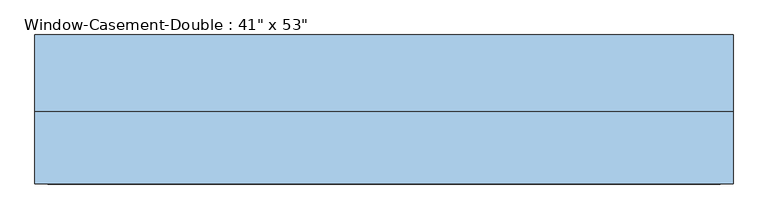
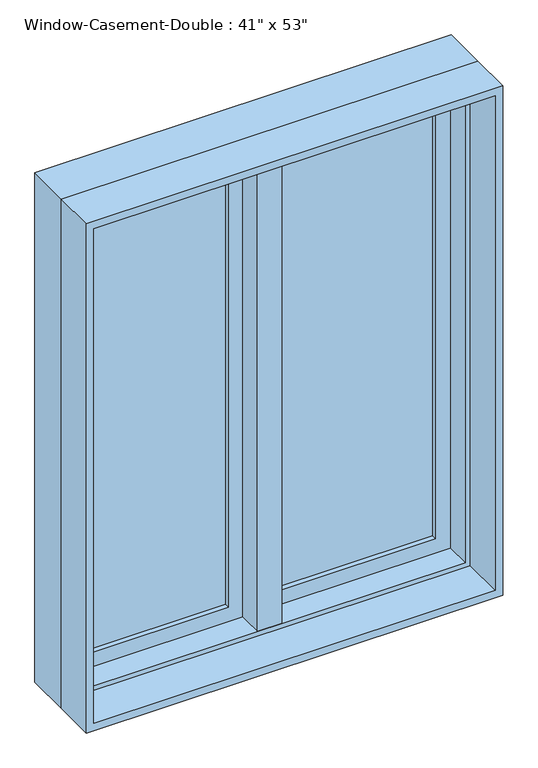
"""IFC4 building model written with IfcOpenShell, lengths in millimetres: window geometry."""

import ifcopenshell
import ifcopenshell.guid

model = None  # the IFC model being written
_history = None  # IfcOwnerHistory: only IFC2X3 demands one
_inside = {}  # id of a spatial element -> (the spatial element, [elements in it])
_under = {}  # id of a project, library or spatial element -> (it, [spatial elements below it])
_declared = {}  # id of a project -> (the project, [libraries it declares])
_typed = {}  # id of a type object -> (the type object, [elements of that type])
_made_of = {}  # id of a material, layer set ... -> (it, [elements and type objects made of it])


def new_model(schema):
    """Start an empty IFC model of exactly this schema.

    Asked for "IFC4X3", IfcOpenShell would pick the latest addendum, in which some entities
    have other attributes; the version numbers below select the first issue.
    IFC2X3 requires an IfcOwnerHistory on every rooted entity: one is made here for all.
    """
    global model, _history
    if schema == "IFC4X3":
        model = ifcopenshell.file(schema_version=(4, 3, 0, 0))
    else:
        model = ifcopenshell.file(schema=schema)
    _inside.clear()
    _under.clear()
    _declared.clear()
    _typed.clear()
    _made_of.clear()
    _history = None
    if model.schema == "IFC2X3":
        org = make("IfcOrganization", Name="unknown")
        user = make(
            "IfcPersonAndOrganization",
            ThePerson=make("IfcPerson", FamilyName="unknown"),
            TheOrganization=org,
        )
        app = make(
            "IfcApplication",
            ApplicationDeveloper=org,
            Version="unknown",
            ApplicationFullName="unknown",
            ApplicationIdentifier="unknown",
        )
        _history = make(
            "IfcOwnerHistory",
            OwningUser=user,
            OwningApplication=app,
            ChangeAction="ADDED",
            CreationDate=0,
        )
    return model


def make(cls, **values):
    """One entity of the class cls with the attributes given. An attribute that is None is left unset."""
    return model.create_entity(
        cls, **{name: value for name, value in values.items() if value is not None}
    )


def rooted(cls, **values):
    """An entity with a GlobalId (a new one), such as an element, a storey or a relation."""
    return make(cls, GlobalId=ifcopenshell.guid.new(), OwnerHistory=_history, **values)


def si_unit(unit_type, name, prefix=None):
    """IfcSIUnit, for example si_unit("LENGTHUNIT", "METRE", prefix="MILLI")."""
    return make("IfcSIUnit", UnitType=unit_type, Prefix=prefix, Name=name)


def assignment(units):
    """IfcUnitAssignment: the units of a project."""
    return None if units is None else make("IfcUnitAssignment", Units=units)


def point(xyz):
    """IfcCartesianPoint."""
    return None if xyz is None else make("IfcCartesianPoint", Coordinates=xyz)


def direction(xyz):
    """IfcDirection."""
    return None if xyz is None else make("IfcDirection", DirectionRatios=xyz)


def frame(location, z_axis=None, x_axis=None):
    """IfcAxis2Placement3D, a coordinate frame: its origin and axes. An axis left out is left unset."""
    return make(
        "IfcAxis2Placement3D",
        Location=point(location),
        Axis=direction(z_axis),
        RefDirection=direction(x_axis),
    )


def origin():
    """The frame at (0, 0, 0) with its axes left unset."""
    return frame((0.0, 0.0, 0.0))


def place(relative_to, where):
    """IfcLocalPlacement: puts the frame where relative to a parent placement (None: the world)."""
    return make(
        "IfcLocalPlacement", PlacementRelTo=relative_to, RelativePlacement=where
    )


def context(
    kind, dimensions, precision=None, world=None, true_north=None, identifier=None
):
    """IfcGeometricRepresentationContext, for example the 3D "Model" context."""
    return make(
        "IfcGeometricRepresentationContext",
        ContextIdentifier=identifier,
        ContextType=kind,
        CoordinateSpaceDimension=dimensions,
        Precision=precision,
        WorldCoordinateSystem=world,
        TrueNorth=true_north,
    )


def project(units=None, contexts=None):
    """IfcProject with its units and contexts."""
    return rooted(
        "IfcProject",
        Name="project",
        RepresentationContexts=contexts,
        UnitsInContext=assignment(units),
    )


def spatial(cls, under=None, at=None, **own):
    """A site, building, storey or space (cls), placed at a placement, below another one or the project."""
    s = rooted(cls, ObjectPlacement=at, **own)
    if under is not None:
        _under.setdefault(under.id(), (under, []))[1].append(s)
    return s


def polyline(points):
    """IfcPolyline through the points."""
    return make("IfcPolyline", Points=[point(p) for p in points])


def outline(outer, holes=None, kind="AREA"):
    """IfcArbitraryClosedProfileDef: a profile drawn as a closed curve; with holes, ...WithVoids."""
    if holes is None:
        return make("IfcArbitraryClosedProfileDef", ProfileType=kind, OuterCurve=outer)
    return make(
        "IfcArbitraryProfileDefWithVoids",
        ProfileType=kind,
        OuterCurve=outer,
        InnerCurves=holes,
    )


def extrude(swept, where, along, depth):
    """IfcExtrudedAreaSolid: the profile swept, set in the frame where, extruded along a direction by depth."""
    return make(
        "IfcExtrudedAreaSolid",
        SweptArea=swept,
        Position=where,
        ExtrudedDirection=direction(along),
        Depth=depth,
    )


def faces_of(points, faces, orient=None, outer=None):
    """IfcFace entities. A face is a list of loops; a loop is a list of indices into points, from 0.

    orient and outer hold one flag for each loop. By default every Orientation is true, the
    first loop of a face is its IfcFaceOuterBound and the others are IfcFaceBound.
    """
    made = []
    for i, loops in enumerate(faces):
        bounds = []
        for j, loop in enumerate(loops):
            is_outer = j == 0 if outer is None else outer[i][j]
            bounds.append(
                make(
                    "IfcFaceOuterBound" if is_outer else "IfcFaceBound",
                    Bound=make("IfcPolyLoop", Polygon=[points[k] for k in loop]),
                    Orientation=True if orient is None else orient[i][j],
                )
            )
        made.append(make("IfcFace", Bounds=bounds))
    return made


def faceted_brep(points, faces, orient=None, outer=None, voids=None):
    """IfcFacetedBrep: a solid bounded by flat faces; with voids (closed shells), ...WithVoids."""
    shared = [point(p) for p in points]
    hull = make("IfcClosedShell", CfsFaces=faces_of(shared, faces, orient, outer))
    if voids is None:
        return make("IfcFacetedBrep", Outer=hull)
    return make(
        "IfcFacetedBrepWithVoids",
        Outer=hull,
        Voids=[
            make(cls, CfsFaces=faces_of(shared, fs, o, b)) for cls, fs, o, b in voids
        ],
    )


def shape(context_of_items, identifier, shape_type, items):
    """IfcShapeRepresentation: the items that make up one representation, for example the "Body"."""
    return make(
        "IfcShapeRepresentation",
        ContextOfItems=context_of_items,
        RepresentationIdentifier=identifier,
        RepresentationType=shape_type,
        Items=items,
    )


def source(mapping_origin, context_of_items, identifier, shape_type, items):
    """IfcRepresentationMap: a shape defined once, which mapped items show again and again."""
    return make(
        "IfcRepresentationMap",
        MappingOrigin=mapping_origin,
        MappedRepresentation=shape(context_of_items, identifier, shape_type, items),
    )


def transform(
    local_origin,
    x_axis=None,
    y_axis=None,
    z_axis=None,
    scale=None,
    scale2=None,
    scale3=None,
    uniform=True,
):
    """IfcCartesianTransformationOperator3D, or its non-uniform kind. x_axis, y_axis, z_axis: its Axis1, 2, 3."""
    if uniform:
        return make(
            "IfcCartesianTransformationOperator3D",
            Axis1=direction(x_axis),
            Axis2=direction(y_axis),
            LocalOrigin=point(local_origin),
            Scale=scale,
            Axis3=direction(z_axis),
        )
    return make(
        "IfcCartesianTransformationOperator3DnonUniform",
        Axis1=direction(x_axis),
        Axis2=direction(y_axis),
        LocalOrigin=point(local_origin),
        Scale=scale,
        Axis3=direction(z_axis),
        Scale2=scale2,
        Scale3=scale3,
    )


def mapped(mapping_source, mapping_target):
    """IfcMappedItem: shows the shape of a source again, moved by a transform."""
    return make(
        "IfcMappedItem", MappingSource=mapping_source, MappingTarget=mapping_target
    )


def made_of(thing, what):
    """Note that an element or type object is made of a material, layer set ...; save() writes the relation."""
    if what is not None:
        _made_of.setdefault(what.id(), (what, []))[1].append(thing)
    return thing


def element(
    cls,
    number,
    at=None,
    inside=None,
    cuts=None,
    type_object=None,
    material=None,
    context=None,
    identifier="Body",
    shape_type=None,
    held_by="IfcProductDefinitionShape",
    body=None,
    shapes=None,
    **own,
):
    """One element of the class cls, such as IfcWall. Its Tag is "e" and its number.

    at: its placement. inside: the storey or other place that contains it. cuts: it is an
    opening in that element (IfcRelVoidsElement). A single representation is given by context,
    identifier, shape_type and body (its items); several are given by shapes. held_by: the class
    of the entity that holds the representations. save() writes the other relations.
    """
    e = rooted(cls, Tag="e%d" % number, ObjectPlacement=at, **own)
    if body is not None:
        shapes = [shape(context, identifier, shape_type, body)]
    if shapes is not None:
        e.Representation = make(held_by, Representations=shapes)
    if inside is not None:
        _inside.setdefault(inside.id(), (inside, []))[1].append(e)
    if cuts is not None:
        rooted(
            "IfcRelVoidsElement", RelatingBuildingElement=cuts, RelatedOpeningElement=e
        )
    if type_object is not None:
        _typed.setdefault(type_object.id(), (type_object, []))[1].append(e)
    return made_of(e, material)


def aggregate(whole, parts):
    """IfcRelAggregates: a whole, such as a stair, and the parts it consists of."""
    return rooted("IfcRelAggregates", RelatingObject=whole, RelatedObjects=parts)


def save(model, path):
    """Write the relations noted so far, then the file.

    IfcRelAggregates (storeys below a building ...), IfcRelContainedInSpatialStructure (elements
    in a storey), IfcRelDefinesByType, IfcRelAssociatesMaterial and IfcRelDeclares: one each for
    every whole, place, type object, material and project.
    """
    for whole, parts in _under.values():
        aggregate(whole, parts)
    for where, things in _inside.values():
        rooted(
            "IfcRelContainedInSpatialStructure",
            RelatedElements=things,
            RelatingStructure=where,
        )
    for kind, things in _typed.values():
        rooted("IfcRelDefinesByType", RelatedObjects=things, RelatingType=kind)
    for what, things in _made_of.values():
        rooted("IfcRelAssociatesMaterial", RelatedObjects=things, RelatingMaterial=what)
    for by, libraries in _declared.values():
        rooted("IfcRelDeclares", RelatingContext=by, RelatedDefinitions=libraries)
    model.write(path)


def window_0de3df1e(model_context):
    return source(origin(), model_context, "Body", "SolidModel", [
        faceted_brep([(9.525, 120.65, 2247.9), (-9.525, 120.65, 2247.9), (-9.525, 69.85, 2247.9), (9.525, 69.85, 2247.9), (9.525, 120.65, 927.1), (9.525, 69.85, 927.1), (-9.525, 69.85, 927.1), (-9.525, 120.65, 927.1), (-9.525, 69.85, 946.15), (-9.525, 69.85, 2228.85), (-30.1625, 69.85, 946.15), (-30.1625, 69.85, 2228.85), (-30.1625, 6.35, 946.15), (-30.1625, 6.35, 2228.85), (30.1625, 6.35, 946.15), (30.1625, 6.35, 2228.85), (30.1625, 69.85, 946.15), (30.1625, 69.85, 2228.85), (9.525, 69.85, 946.15), (9.525, 69.85, 2228.85)], [[[0, 1, 2, 3]], [[4, 5, 6, 7]], [[1, 0, 4, 7]], [[2, 1, 7, 6, 8, 9]], [[9, 8, 10, 11]], [[11, 10, 12, 13]], [[13, 12, 14, 15]], [[15, 14, 16, 17]], [[17, 16, 18, 19]], [[0, 3, 19, 18, 5, 4]], [[18, 8, 6, 5]], [[9, 19, 3, 2]], [[8, 18, 16, 14, 12, 10]], [[19, 9, 11, 13, 15, 17]]]),
        extrude(outline(polyline([(-66.675, 101.6), (-66.675, 95.25), (-450.85, 95.25), (-450.85, 101.6), (-66.675, 101.6)])), frame((0.0, 0.0, 984.25), z_axis=(0.0, 0.0, 1.0), x_axis=(1.0, 0.0, 0.0)), (0.0, 0.0, 1.0), 1206.5),
        extrude(outline(polyline([(-450.85, 82.55), (-450.85, 88.9), (-66.675, 88.9), (-66.675, 82.55), (-450.85, 82.55)])), frame((0.0, 0.0, 984.25), z_axis=(0.0, 0.0, 1.0), x_axis=(1.0, 0.0, 0.0)), (0.0, 0.0, 1.0), 1206.5),
        extrude(outline(polyline([(450.85, 101.6), (450.85, 95.25), (66.675, 95.25), (66.675, 101.6), (450.85, 101.6)])), frame((0.0, 0.0, 984.25), z_axis=(0.0, 0.0, 1.0), x_axis=(1.0, 0.0, 0.0)), (0.0, 0.0, 1.0), 1206.5),
        extrude(outline(polyline([(66.675, 82.55), (66.675, 88.9), (450.85, 88.9), (450.85, 82.55), (66.675, 82.55)])), frame((0.0, 0.0, 984.25), z_axis=(0.0, 0.0, 1.0), x_axis=(1.0, 0.0, 0.0)), (0.0, 0.0, 1.0), 1206.5),
        extrude(outline(polyline([(2247.9, -508.0), (927.1, -508.0), (927.1, -9.525), (2247.9, -9.525), (2247.9, -508.0)]), holes=[polyline([(2190.75, -66.675), (984.25, -66.675), (984.25, -450.85), (2190.75, -450.85), (2190.75, -66.675)])]), frame((0.0, 69.85, 0.0), z_axis=(0.0, 1.0, 0.0), x_axis=(0.0, 0.0, 1.0)), (0.0, 0.0, 1.0), 44.45),
        extrude(outline(polyline([(927.1, 508.0), (2247.9, 508.0), (2247.9, 9.525), (927.1, 9.525), (927.1, 508.0)]), holes=[polyline([(984.25, 66.675), (2190.75, 66.675), (2190.75, 450.85), (984.25, 450.85), (984.25, 66.675)])]), frame((0.0, 69.85, 0.0), z_axis=(0.0, 1.0, 0.0), x_axis=(0.0, 0.0, 1.0)), (0.0, 0.0, 1.0), 44.45),
        extrude(outline(polyline([(2260.6, -520.7), (914.4, -520.7), (914.4, 520.7), (2260.6, 520.7), (2260.6, -520.7)]), holes=[polyline([(2241.55, 501.65), (933.45, 501.65), (933.45, -501.65), (2241.55, -501.65), (2241.55, 501.65)])]), frame((0.0, -101.6, 0.0), z_axis=(0.0, 1.0, 0.0), x_axis=(0.0, 0.0, 1.0)), (0.0, 0.0, 1.0), 107.95),
        faceted_brep([(488.95, 69.85, 2228.85), (488.95, 6.35, 2228.85), (-488.95, 6.35, 2228.85), (-488.95, 69.85, 2228.85), (508.0, 120.65, 2247.9), (508.0, 69.85, 2247.9), (-508.0, 69.85, 2247.9), (-508.0, 120.65, 2247.9), (520.7, 6.35, 2260.6), (520.7, 120.65, 2260.6), (-520.7, 120.65, 2260.6), (-520.7, 6.35, 2260.6), (-488.95, 6.35, 946.15), (-488.95, 69.85, 946.15), (-508.0, 69.85, 927.1), (-508.0, 120.65, 927.1), (-520.7, 120.65, 914.4), (-520.7, 6.35, 914.4), (488.95, 6.35, 946.15), (488.95, 69.85, 946.15), (508.0, 69.85, 927.1), (508.0, 120.65, 927.1), (520.7, 120.65, 914.4), (520.7, 6.35, 914.4)], [[[0, 1, 2, 3]], [[4, 5, 6, 7]], [[8, 9, 10, 11]], [[3, 2, 12, 13]], [[7, 6, 14, 15]], [[11, 10, 16, 17]], [[13, 12, 18, 19]], [[15, 14, 20, 21]], [[17, 16, 22, 23]], [[11, 17, 23, 8], [1, 18, 12, 2]], [[19, 18, 1, 0]], [[5, 20, 14, 6], [3, 13, 19, 0]], [[21, 20, 5, 4]], [[23, 22, 9, 8]], [[9, 22, 16, 10], [7, 15, 21, 4]]]),
    ])


if __name__ == "__main__":
    model = new_model("IFC4")
    model_context = context("Model", 3, world=origin())
    ifc_project = project(units=[si_unit("LENGTHUNIT", "METRE", prefix="MILLI")], contexts=[model_context])
    site = spatial("IfcSite", under=ifc_project)
    building = spatial("IfcBuilding", under=site)
    placement = place(None, origin())
    window_shape = window_0de3df1e(model_context)
    element("IfcWindow", 1, ObjectType="Window-Casement-Double : 41\" x 53\"", at=placement, inside=building, context=model_context, shape_type="MappedRepresentation", body=[
        mapped(window_shape, transform((0.0, 0.0, 0.0), x_axis=(1.0, 0.0, 0.0), y_axis=(0.0, 1.0, 0.0), z_axis=(0.0, 0.0, 1.0))),
    ])
    save(model, "model.ifc")

# Revit data of these elements
# Type "Window-Casement-Double : 41\" x 53\""
#   Type Mark = "60"
#   Fire Rating = "0.5h"
#   Assembly Code = "B2020100"
#   Analytic Construction = "Double glazing - domestic"
#   Frame Extension [instance default] = 0' - 0 1/4"
#   Window Inset [instance default] = 0' - 0"
#   Wall Thickness [instance default] = 0' - 6"
#   Interior Wall Closure [instance default] = 0' - 2 1/4"
#   Half Width = 1' - 8 1/2"
#   Visual Light Transmittance = 0.81
#   Thermal Resistance (R) = 1.8146 (h·ft²·°F)/BTU
#   Solar Heat Gain Coefficient = 0.76
#   Rough Width = 3' - 5 1/2"
#   Rough Height = 4' - 5 1/2"
#   Height = 4' - 5"
#   Heat Transfer Coefficient (U) = 0.5511 BTU/(h·ft²·°F)
#   Exterior Wall Closure [instance default] = 0' - 1 1/4"
#   Extension Jamb [instance default] = 0' - 2 1/4"
#   Default Sill Height = 3' - 0"
#   Width = 3' - 5"
#   Define Thermal Properties by = 0
#   Muntin Visibility = yes
#   Interior Trim Visibility [instance default] = yes
#   Exterior Trim Visibility [instance default] = yes
#   Extension Jamb Visibility [instance default] = yes
#   Interior Trim Material = Wood - Stained
#   Muntin Pattern = Muntin Pattern_2x2 : Muntin Pattern_2x2
#   Interior Trim = Trim-Window-Interior-Flat : Picture Frame
#   Interior Frame Material = Wood - Stained
#   Glass Panel Material = Glass
#   Exterior Trim Material = Clad - White
#   Exterior Trim = Trim-Window-Exterior-Flat : with Sill
#   Exterior Frame Material = Clad - White
#   Wall Closure = (empty or 0)
# Element 1 (IfcWindow, "Window-Casement-Double : 41\" x 53\"")
#   Wall Thickness = 0' - 8"
#   Extension Jamb = 0' - 4 1/4"
#   Materials on its faces: "Wood - Stained", "Glass", "Clad - White"
# Materials
#   "Wood - Stained": class "Wood", colour RGB 224 178 126, transparency 0, Cost = 0
#   "Glass": class "Glass", colour RGB 236 240 239, transparency 0.5, Description = "Soda Lime Glass", Cost = 0
#   "Clad - White": class "Wood", colour RGB 216 216 204, transparency 0, Cost = 0
